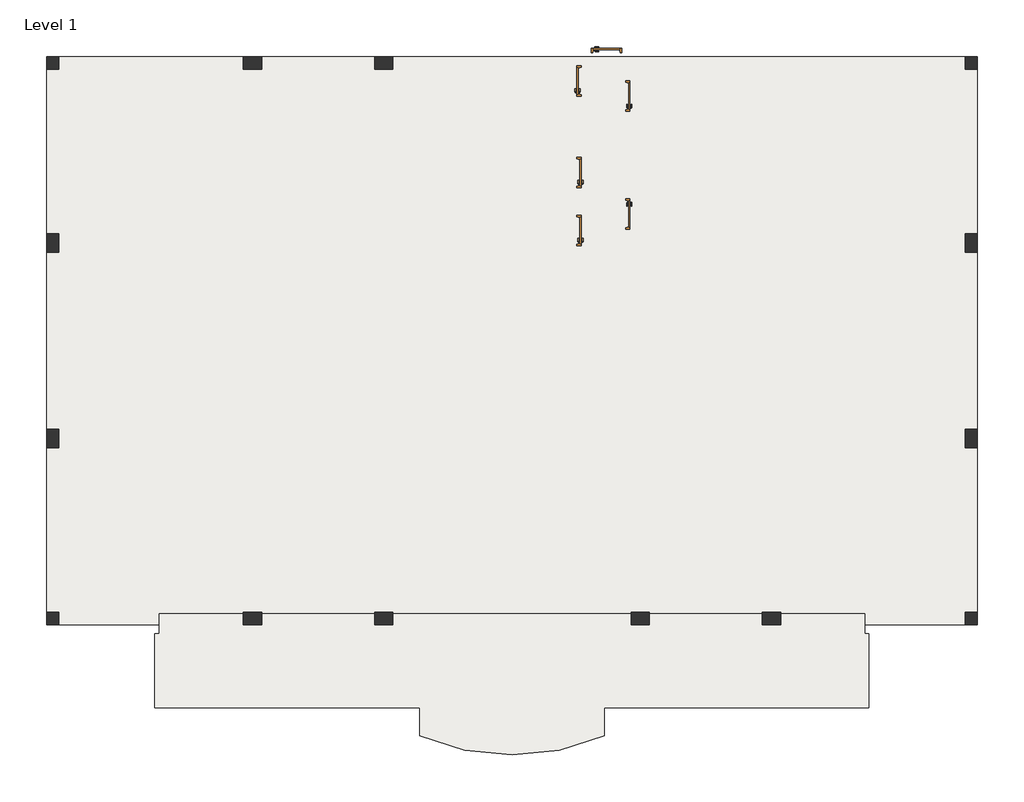
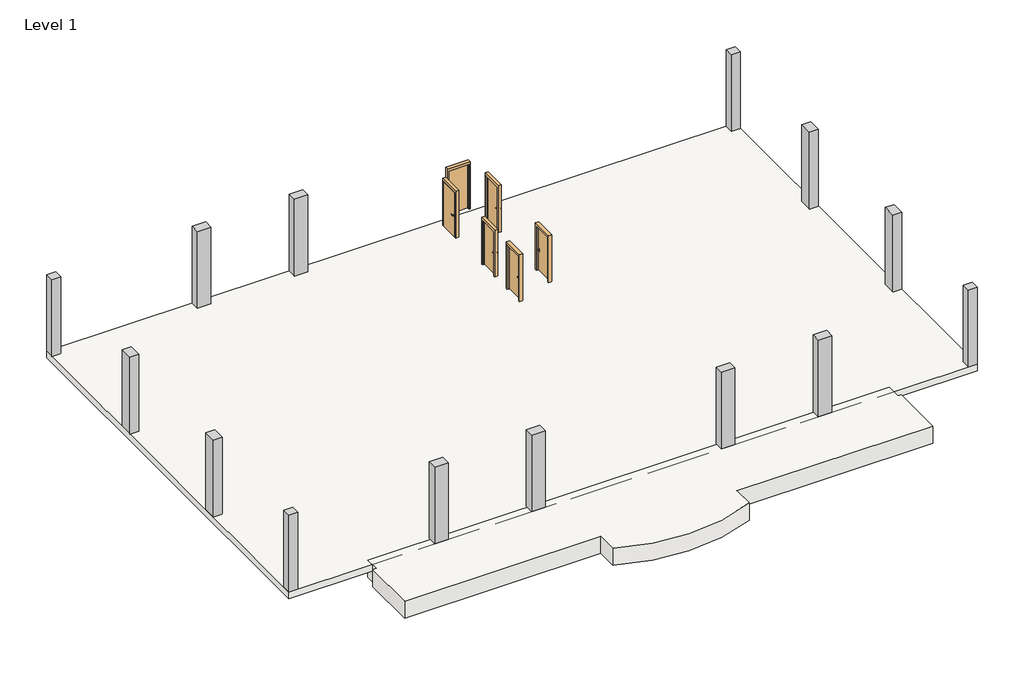
# One storey: 14 columns, 6 doors, 2 slabs.
"""IFC4 building model written with IfcOpenShell, lengths in millimetres."""

import ifcopenshell
import ifcopenshell.guid

model = None  # the IFC model being written
_history = None  # IfcOwnerHistory: only IFC2X3 demands one
_inside = {}  # id of a spatial element -> (the spatial element, [elements in it])
_under = {}  # id of a project, library or spatial element -> (it, [spatial elements below it])
_declared = {}  # id of a project -> (the project, [libraries it declares])
_typed = {}  # id of a type object -> (the type object, [elements of that type])
_made_of = {}  # id of a material, layer set ... -> (it, [elements and type objects made of it])


def new_model(schema):
    """Start an empty IFC model of exactly this schema.

    Asked for "IFC4X3", IfcOpenShell would pick the latest addendum, in which some entities
    have other attributes; the version numbers below select the first issue.
    IFC2X3 requires an IfcOwnerHistory on every rooted entity: one is made here for all.
    """
    global model, _history
    if schema == "IFC4X3":
        model = ifcopenshell.file(schema_version=(4, 3, 0, 0))
    else:
        model = ifcopenshell.file(schema=schema)
    _inside.clear()
    _under.clear()
    _declared.clear()
    _typed.clear()
    _made_of.clear()
    _history = None
    if model.schema == "IFC2X3":
        org = make("IfcOrganization", Name="unknown")
        user = make(
            "IfcPersonAndOrganization",
            ThePerson=make("IfcPerson", FamilyName="unknown"),
            TheOrganization=org,
        )
        app = make(
            "IfcApplication",
            ApplicationDeveloper=org,
            Version="unknown",
            ApplicationFullName="unknown",
            ApplicationIdentifier="unknown",
        )
        _history = make(
            "IfcOwnerHistory",
            OwningUser=user,
            OwningApplication=app,
            ChangeAction="ADDED",
            CreationDate=0,
        )
    return model


def make(cls, **values):
    """One entity of the class cls with the attributes given. An attribute that is None is left unset."""
    return model.create_entity(
        cls, **{name: value for name, value in values.items() if value is not None}
    )


def rooted(cls, **values):
    """An entity with a GlobalId (a new one), such as an element, a storey or a relation."""
    return make(cls, GlobalId=ifcopenshell.guid.new(), OwnerHistory=_history, **values)


def si_unit(unit_type, name, prefix=None):
    """IfcSIUnit, for example si_unit("LENGTHUNIT", "METRE", prefix="MILLI")."""
    return make("IfcSIUnit", UnitType=unit_type, Prefix=prefix, Name=name)


def assignment(units):
    """IfcUnitAssignment: the units of a project."""
    return None if units is None else make("IfcUnitAssignment", Units=units)


def point(xyz):
    """IfcCartesianPoint."""
    return None if xyz is None else make("IfcCartesianPoint", Coordinates=xyz)


def direction(xyz):
    """IfcDirection."""
    return None if xyz is None else make("IfcDirection", DirectionRatios=xyz)


def frame(location, z_axis=None, x_axis=None):
    """IfcAxis2Placement3D, a coordinate frame: its origin and axes. An axis left out is left unset."""
    return make(
        "IfcAxis2Placement3D",
        Location=point(location),
        Axis=direction(z_axis),
        RefDirection=direction(x_axis),
    )


def frame_2d(location, x_axis=None):
    """IfcAxis2Placement2D, a coordinate frame in the plane: its origin and x axis."""
    return make(
        "IfcAxis2Placement2D", Location=point(location), RefDirection=direction(x_axis)
    )


def origin():
    """The frame at (0, 0, 0) with its axes left unset."""
    return frame((0.0, 0.0, 0.0))


def origin_with_axes():
    """The frame at (0, 0, 0) with the z axis (0, 0, 1) and the x axis (1, 0, 0) written out."""
    return frame((0.0, 0.0, 0.0), z_axis=(0.0, 0.0, 1.0), x_axis=(1.0, 0.0, 0.0))


def place(relative_to, where):
    """IfcLocalPlacement: puts the frame where relative to a parent placement (None: the world)."""
    return make(
        "IfcLocalPlacement", PlacementRelTo=relative_to, RelativePlacement=where
    )


def context(
    kind, dimensions, precision=None, world=None, true_north=None, identifier=None
):
    """IfcGeometricRepresentationContext, for example the 3D "Model" context."""
    return make(
        "IfcGeometricRepresentationContext",
        ContextIdentifier=identifier,
        ContextType=kind,
        CoordinateSpaceDimension=dimensions,
        Precision=precision,
        WorldCoordinateSystem=world,
        TrueNorth=true_north,
    )


def project(units=None, contexts=None):
    """IfcProject with its units and contexts."""
    return rooted(
        "IfcProject",
        Name="project",
        RepresentationContexts=contexts,
        UnitsInContext=assignment(units),
    )


def spatial(cls, under=None, at=None, **own):
    """A site, building, storey or space (cls), placed at a placement, below another one or the project."""
    s = rooted(cls, ObjectPlacement=at, **own)
    if under is not None:
        _under.setdefault(under.id(), (under, []))[1].append(s)
    return s


def polyline(points):
    """IfcPolyline through the points."""
    return make("IfcPolyline", Points=[point(p) for p in points])


def circle_curve(where, radius):
    """IfcCircle in the frame where."""
    return make("IfcCircle", Position=where, Radius=radius)


def ellipse_curve(where, semi_axis1, semi_axis2):
    """IfcEllipse in the frame where."""
    return make(
        "IfcEllipse", Position=where, SemiAxis1=semi_axis1, SemiAxis2=semi_axis2
    )


def trimmed(basis, trim1, trim2, sense, master):
    """IfcTrimmedCurve: the piece of a basis curve between two trims."""
    return make(
        "IfcTrimmedCurve",
        BasisCurve=basis,
        Trim1=trim1,
        Trim2=trim2,
        SenseAgreement=sense,
        MasterRepresentation=master,
    )


def segment(curve, same_sense, transition):
    """IfcCompositeCurveSegment."""
    return make(
        "IfcCompositeCurveSegment",
        Transition=transition,
        SameSense=same_sense,
        ParentCurve=curve,
    )


def composite_curve(segments, self_intersect=None):
    """IfcCompositeCurve: segments joined end to end."""
    return make("IfcCompositeCurve", Segments=segments, SelfIntersect=self_intersect)


def outline(outer, holes=None, kind="AREA"):
    """IfcArbitraryClosedProfileDef: a profile drawn as a closed curve; with holes, ...WithVoids."""
    if holes is None:
        return make("IfcArbitraryClosedProfileDef", ProfileType=kind, OuterCurve=outer)
    return make(
        "IfcArbitraryProfileDefWithVoids",
        ProfileType=kind,
        OuterCurve=outer,
        InnerCurves=holes,
    )


def extrude(swept, where, along, depth):
    """IfcExtrudedAreaSolid: the profile swept, set in the frame where, extruded along a direction by depth."""
    return make(
        "IfcExtrudedAreaSolid",
        SweptArea=swept,
        Position=where,
        ExtrudedDirection=direction(along),
        Depth=depth,
    )


def faces_of(points, faces, orient=None, outer=None):
    """IfcFace entities. A face is a list of loops; a loop is a list of indices into points, from 0.

    orient and outer hold one flag for each loop. By default every Orientation is true, the
    first loop of a face is its IfcFaceOuterBound and the others are IfcFaceBound.
    """
    made = []
    for i, loops in enumerate(faces):
        bounds = []
        for j, loop in enumerate(loops):
            is_outer = j == 0 if outer is None else outer[i][j]
            bounds.append(
                make(
                    "IfcFaceOuterBound" if is_outer else "IfcFaceBound",
                    Bound=make("IfcPolyLoop", Polygon=[points[k] for k in loop]),
                    Orientation=True if orient is None else orient[i][j],
                )
            )
        made.append(make("IfcFace", Bounds=bounds))
    return made


def faceted_brep(points, faces, orient=None, outer=None, voids=None):
    """IfcFacetedBrep: a solid bounded by flat faces; with voids (closed shells), ...WithVoids."""
    shared = [point(p) for p in points]
    hull = make("IfcClosedShell", CfsFaces=faces_of(shared, faces, orient, outer))
    if voids is None:
        return make("IfcFacetedBrep", Outer=hull)
    return make(
        "IfcFacetedBrepWithVoids",
        Outer=hull,
        Voids=[
            make(cls, CfsFaces=faces_of(shared, fs, o, b)) for cls, fs, o, b in voids
        ],
    )


def shape(context_of_items, identifier, shape_type, items):
    """IfcShapeRepresentation: the items that make up one representation, for example the "Body"."""
    return make(
        "IfcShapeRepresentation",
        ContextOfItems=context_of_items,
        RepresentationIdentifier=identifier,
        RepresentationType=shape_type,
        Items=items,
    )


def source(mapping_origin, context_of_items, identifier, shape_type, items):
    """IfcRepresentationMap: a shape defined once, which mapped items show again and again."""
    return make(
        "IfcRepresentationMap",
        MappingOrigin=mapping_origin,
        MappedRepresentation=shape(context_of_items, identifier, shape_type, items),
    )


def transform(
    local_origin,
    x_axis=None,
    y_axis=None,
    z_axis=None,
    scale=None,
    scale2=None,
    scale3=None,
    uniform=True,
):
    """IfcCartesianTransformationOperator3D, or its non-uniform kind. x_axis, y_axis, z_axis: its Axis1, 2, 3."""
    if uniform:
        return make(
            "IfcCartesianTransformationOperator3D",
            Axis1=direction(x_axis),
            Axis2=direction(y_axis),
            LocalOrigin=point(local_origin),
            Scale=scale,
            Axis3=direction(z_axis),
        )
    return make(
        "IfcCartesianTransformationOperator3DnonUniform",
        Axis1=direction(x_axis),
        Axis2=direction(y_axis),
        LocalOrigin=point(local_origin),
        Scale=scale,
        Axis3=direction(z_axis),
        Scale2=scale2,
        Scale3=scale3,
    )


def mapped(mapping_source, mapping_target):
    """IfcMappedItem: shows the shape of a source again, moved by a transform."""
    return make(
        "IfcMappedItem", MappingSource=mapping_source, MappingTarget=mapping_target
    )


def made_of(thing, what):
    """Note that an element or type object is made of a material, layer set ...; save() writes the relation."""
    if what is not None:
        _made_of.setdefault(what.id(), (what, []))[1].append(thing)
    return thing


def element(
    cls,
    number,
    at=None,
    inside=None,
    cuts=None,
    type_object=None,
    material=None,
    context=None,
    identifier="Body",
    shape_type=None,
    held_by="IfcProductDefinitionShape",
    body=None,
    shapes=None,
    **own,
):
    """One element of the class cls, such as IfcWall. Its Tag is "e" and its number.

    at: its placement. inside: the storey or other place that contains it. cuts: it is an
    opening in that element (IfcRelVoidsElement). A single representation is given by context,
    identifier, shape_type and body (its items); several are given by shapes. held_by: the class
    of the entity that holds the representations. save() writes the other relations.
    """
    e = rooted(cls, Tag="e%d" % number, ObjectPlacement=at, **own)
    if body is not None:
        shapes = [shape(context, identifier, shape_type, body)]
    if shapes is not None:
        e.Representation = make(held_by, Representations=shapes)
    if inside is not None:
        _inside.setdefault(inside.id(), (inside, []))[1].append(e)
    if cuts is not None:
        rooted(
            "IfcRelVoidsElement", RelatingBuildingElement=cuts, RelatedOpeningElement=e
        )
    if type_object is not None:
        _typed.setdefault(type_object.id(), (type_object, []))[1].append(e)
    return made_of(e, material)


def aggregate(whole, parts):
    """IfcRelAggregates: a whole, such as a stair, and the parts it consists of."""
    return rooted("IfcRelAggregates", RelatingObject=whole, RelatedObjects=parts)


def save(model, path):
    """Write the relations noted so far, then the file.

    IfcRelAggregates (storeys below a building ...), IfcRelContainedInSpatialStructure (elements
    in a storey), IfcRelDefinesByType, IfcRelAssociatesMaterial and IfcRelDeclares: one each for
    every whole, place, type object, material and project.
    """
    for whole, parts in _under.values():
        aggregate(whole, parts)
    for where, things in _inside.values():
        rooted(
            "IfcRelContainedInSpatialStructure",
            RelatedElements=things,
            RelatingStructure=where,
        )
    for kind, things in _typed.values():
        rooted("IfcRelDefinesByType", RelatedObjects=things, RelatingType=kind)
    for what, things in _made_of.values():
        rooted("IfcRelAssociatesMaterial", RelatedObjects=things, RelatingMaterial=what)
    for by, libraries in _declared.values():
        rooted("IfcRelDeclares", RelatingContext=by, RelatedDefinitions=libraries)
    model.write(path)


def plane_surface(at):
    """IfcPlane: the flat surface through the origin of the frame at, square to its z axis."""
    return make("IfcPlane", Position=at)


def cylinder_surface(at, radius):
    """IfcCylindricalSurface: all points at the distance radius from the z axis of the frame at."""
    return make("IfcCylindricalSurface", Position=at, Radius=radius)


def revolved_surface(curve, axis_point, axis_direction):
    """IfcSurfaceOfRevolution: the curve turned about the line through axis_point along axis_direction."""
    return make(
        "IfcSurfaceOfRevolution",
        SweptCurve=make("IfcArbitraryOpenProfileDef", ProfileType="CURVE", Curve=curve),
        AxisPosition=make("IfcAxis1Placement", Location=point(axis_point), Axis=direction(axis_direction)),
    )


def advanced_brep(points, edges, surfaces, faces):
    """IfcAdvancedBrep: a solid bounded by faces that lie on surfaces and meet in shared edges.

    An edge is (start, end): straight between two places in points (the first is 0);
    or (start, end, curve); or (start, end, curve, False) where it runs against its curve.
    A face is (place in surfaces, loops), or (place, loops, False) where it looks against
    its surface's normal. A loop lists edges by number (the first is 1), with a minus sign
    where the edge is run from its end to its start. The first loop is the outer one.
    """
    corners = [point(p) for p in points]
    vertices = [make("IfcVertexPoint", VertexGeometry=c) for c in corners]
    made = []
    for start, end, *more in edges:
        made.append(
            make(
                "IfcEdgeCurve",
                EdgeStart=vertices[start],
                EdgeEnd=vertices[end],
                EdgeGeometry=more[0] if more else make("IfcPolyline", Points=[corners[start], corners[end]]),
                SameSense=more[1] if len(more) > 1 else True,
            )
        )
    hull = []
    for where, loops, *sense in faces:
        bounds = []
        for j, loop in enumerate(loops):
            ring = [make("IfcOrientedEdge", EdgeElement=made[abs(k) - 1], Orientation=k > 0) for k in loop]
            bounds.append(
                make(
                    "IfcFaceOuterBound" if j == 0 else "IfcFaceBound",
                    Bound=make("IfcEdgeLoop", EdgeList=ring),
                    Orientation=True,
                )
            )
        hull.append(make("IfcAdvancedFace", Bounds=bounds, FaceSurface=surfaces[where], SameSense=sense[0] if sense else True))
    return make("IfcAdvancedBrep", Outer=make("IfcClosedShell", CfsFaces=hull))


def door_e56c0533(model_context):
    return source(origin(), model_context, "Body", "SolidModel", [
        advanced_brep(
        [(-392.190625, 76.1375, 1016.0), (-372.190625, 76.1375, 1016.0), (-372.190625, 46.1375, 1016.0), (-392.190625, 46.1375, 1016.0), (-367.190625, 41.1375, 1016.0), (-367.190625, 21.1375, 1016.0), (-262.190625, 21.1375, 1016.0), (-262.190625, 41.1375, 1016.0)],
        [
            (0, 1, circle_curve(frame((-382.190625, 76.1375, 1016.0), z_axis=(0.0, 1.0, 0.0), x_axis=(1.0, 0.0, 0.0)), 10.0)),
            (1, 0, circle_curve(frame((-382.190625, 76.1375, 1016.0), z_axis=(0.0, 1.0, 0.0), x_axis=(1.0, 0.0, 0.0)), 10.0)),
            (1, 2),
            (2, 3, circle_curve(frame((-382.190625, 46.1375, 1016.0), z_axis=(0.0, 1.0, 0.0), x_axis=(1.0, 0.0, 0.0)), 10.0)),
            (3, 0),
            (3, 2, circle_curve(frame((-382.190625, 46.1375, 1016.0), z_axis=(0.0, 1.0, 0.0), x_axis=(1.0, 0.0, 0.0)), 10.0)),
            (4, 5, circle_curve(frame((-367.190625, 31.1375, 1016.0), z_axis=(-1.0, 0.0, 0.0), x_axis=(0.0, 1.0, 0.0)), 10.0)),
            (5, 3, circle_curve(frame((-367.190625, 46.1375, 1016.0), z_axis=(0.0, 0.0, -1.0), x_axis=(-1.0, 0.0, 0.0)), 25.0)),
            (2, 4, circle_curve(frame((-367.190625, 46.1375, 1016.0), z_axis=(0.0, 0.0, 1.0), x_axis=(-1.0, 0.0, 0.0)), 5.0)),
            (5, 4, circle_curve(frame((-367.190625, 31.1375, 1016.0), z_axis=(-1.0, 0.0, 0.0), x_axis=(0.0, 1.0, 0.0)), 10.0)),
            (6, 7, circle_curve(frame((-262.190625, 31.1375, 1016.0), z_axis=(1.0, 0.0, 0.0), x_axis=(0.0, 1.0, 0.0)), 10.0)),
            (7, 6, circle_curve(frame((-262.190625, 31.1375, 1016.0), z_axis=(1.0, 0.0, 0.0), x_axis=(0.0, 1.0, 0.0)), 10.0)),
            (4, 7),
            (6, 5),
        ],
        [
            plane_surface(frame((-382.190625, 76.1375, 1016.0), z_axis=(0.0, 1.0, 0.0), x_axis=(0.0, 0.0, 1.0))),
            cylinder_surface(frame((-382.190625, 76.1375, 1016.0), z_axis=(0.0, 1.0, 0.0), x_axis=(1.0, 0.0, 0.0)), 10.0),
            revolved_surface(trimmed(ellipse_curve(frame((-382.190625, 46.1375, 1016.0), z_axis=(0.0, -1.0, 0.0), x_axis=(1.0, 0.0, 0.0)), 10.0, 10.0), [point((-392.190625, 46.1375, 1016.0))], [point((-372.190625, 46.1375, 1016.0))], True, "CARTESIAN"), (-367.190625, 46.1375, 1016.0), (0.0, 0.0, -1.0)),
            revolved_surface(trimmed(ellipse_curve(frame((-382.190625, 46.1375, 1016.0), z_axis=(0.0, -1.0, 0.0), x_axis=(1.0, 0.0, 0.0)), 10.0, 10.0), [point((-372.190625, 46.1375, 1016.0))], [point((-392.190625, 46.1375, 1016.0))], True, "CARTESIAN"), (-367.190625, 46.1375, 1016.0), (0.0, 0.0, -1.0)),
            plane_surface(frame((-262.190625, 31.1375, 1016.0), z_axis=(1.0, 0.0, 0.0), x_axis=(0.0, 0.0, 1.0))),
            cylinder_surface(frame((-367.190625, 31.1375, 1016.0), z_axis=(-1.0, 0.0, 0.0), x_axis=(0.0, 1.0, 0.0)), 10.0),
        ],
        [
            (0, [[1, 2]]),
            (1, [[3, 4, 5, -2]]),
            (1, [[-5, 6, -3, -1]]),
            (2, [[7, 8, -4, 9]]),
            (3, [[10, -9, -6, -8]]),
            (4, [[11, 12]]),
            (5, [[13, -11, 14, -7]]),
            (5, [[-14, -12, -13, -10]]),
        ],
    ),
        extrude(outline(composite_curve([segment(trimmed(circle_curve(frame_2d((1016.0, -384.690625)), 30.0), [point((1016.0, -414.690625))], [point((1016.0, -354.690625))], False, "CARTESIAN"), True, "CONTINUOUS"), segment(trimmed(circle_curve(frame_2d((1016.0, -384.690625)), 30.0), [point((1016.0, -354.690625))], [point((1016.0, -414.690625))], False, "CARTESIAN"), True, "CONTINUOUS")], self_intersect=False)), frame((0.0, 76.1375, 0.0), z_axis=(0.0, 1.0, 0.0), x_axis=(0.0, 0.0, 1.0)), (0.0, 0.0, 1.0), 8.0),
        advanced_brep(
        [(-392.190625, 136.5875, 1016.0), (-372.190625, 136.5875, 1016.0), (-392.190625, 166.5875, 1016.0), (-372.190625, 166.5875, 1016.0), (-367.190625, 171.5875, 1016.0), (-367.190625, 191.5875, 1016.0), (-262.190625, 191.5875, 1016.0), (-262.190625, 171.5875, 1016.0)],
        [
            (0, 1, circle_curve(frame((-382.190625, 136.5875, 1016.0), z_axis=(0.0, -1.0, 0.0), x_axis=(1.0, 0.0, 0.0)), 10.0)),
            (1, 0, circle_curve(frame((-382.190625, 136.5875, 1016.0), z_axis=(0.0, -1.0, 0.0), x_axis=(1.0, 0.0, 0.0)), 10.0)),
            (0, 2),
            (2, 3, circle_curve(frame((-382.190625, 166.5875, 1016.0), z_axis=(0.0, -1.0, 0.0), x_axis=(1.0, 0.0, 0.0)), 10.0)),
            (3, 1),
            (3, 2, circle_curve(frame((-382.190625, 166.5875, 1016.0), z_axis=(0.0, -1.0, 0.0), x_axis=(1.0, 0.0, 0.0)), 10.0)),
            (4, 3, circle_curve(frame((-367.190625, 166.5875, 1016.0), z_axis=(0.0, 0.0, 1.0), x_axis=(-1.0, 0.0, 0.0)), 5.0)),
            (2, 5, circle_curve(frame((-367.190625, 166.5875, 1016.0), z_axis=(0.0, 0.0, -1.0), x_axis=(-1.0, 0.0, 0.0)), 25.0)),
            (5, 4, circle_curve(frame((-367.190625, 181.5875, 1016.0), z_axis=(-1.0, 0.0, 0.0), x_axis=(0.0, -1.0, 0.0)), 10.0)),
            (4, 5, circle_curve(frame((-367.190625, 181.5875, 1016.0), z_axis=(-1.0, 0.0, 0.0), x_axis=(0.0, -1.0, 0.0)), 10.0)),
            (6, 7, circle_curve(frame((-262.190625, 181.5875, 1016.0), z_axis=(1.0, 0.0, 0.0), x_axis=(0.0, -1.0, 0.0)), 10.0)),
            (7, 6, circle_curve(frame((-262.190625, 181.5875, 1016.0), z_axis=(1.0, 0.0, 0.0), x_axis=(0.0, -1.0, 0.0)), 10.0)),
            (5, 6),
            (7, 4),
        ],
        [
            plane_surface(frame((-382.190625, 136.5875, 1016.0), z_axis=(0.0, -1.0, 0.0), x_axis=(0.0, 0.0, 1.0))),
            cylinder_surface(frame((-382.190625, 136.5875, 1016.0), z_axis=(0.0, -1.0, 0.0), x_axis=(1.0, 0.0, 0.0)), 10.0),
            revolved_surface(trimmed(ellipse_curve(frame((-382.190625, 166.5875, 1016.0), z_axis=(0.0, -1.0, 0.0), x_axis=(1.0, 0.0, 0.0)), 10.0, 10.0), [point((-392.190625, 166.5875, 1016.0))], [point((-372.190625, 166.5875, 1016.0))], True, "CARTESIAN"), (-367.190625, 166.5875, 1016.0), (0.0, 0.0, -1.0)),
            revolved_surface(trimmed(ellipse_curve(frame((-382.190625, 166.5875, 1016.0), z_axis=(0.0, -1.0, 0.0), x_axis=(1.0, 0.0, 0.0)), 10.0, 10.0), [point((-372.190625, 166.5875, 1016.0))], [point((-392.190625, 166.5875, 1016.0))], True, "CARTESIAN"), (-367.190625, 166.5875, 1016.0), (0.0, 0.0, -1.0)),
            plane_surface(frame((-262.190625, 181.5875, 1016.0), z_axis=(1.0, 0.0, 0.0), x_axis=(0.0, 0.0, 1.0))),
            cylinder_surface(frame((-367.190625, 181.5875, 1016.0), z_axis=(-1.0, 0.0, 0.0), x_axis=(0.0, -1.0, 0.0)), 10.0),
        ],
        [
            (0, [[1, 2]]),
            (1, [[-1, 3, 4, 5]]),
            (1, [[-2, -5, 6, -3]]),
            (2, [[7, -4, 8, 9]]),
            (3, [[-8, -6, -7, 10]]),
            (4, [[11, 12]]),
            (5, [[-9, 13, -12, 14]]),
            (5, [[-10, -14, -11, -13]]),
        ],
    ),
        extrude(outline(composite_curve([segment(trimmed(circle_curve(frame_2d((1016.0, -384.690625)), 30.0), [point((1016.0, -414.690625))], [point((1016.0, -354.690625))], False, "CARTESIAN"), True, "CONTINUOUS"), segment(trimmed(circle_curve(frame_2d((1016.0, -384.690625)), 30.0), [point((1016.0, -354.690625))], [point((1016.0, -414.690625))], False, "CARTESIAN"), True, "CONTINUOUS")], self_intersect=False)), frame((0.0, 128.5875, 0.0), z_axis=(0.0, 1.0, 0.0), x_axis=(0.0, 0.0, 1.0)), (0.0, 0.0, 1.0), 8.0),
        faceted_brep([(457.2, 79.375, 0.0), (457.2, 128.5875, 0.0), (508.0, 128.5875, 0.0), (508.0, -17.4625, 0.0), (457.2, -17.4625, 0.0), (457.2, 31.75, 0.0), (441.325, 31.75, 0.0), (441.325, 79.375, 0.0), (457.2, 79.375, 2133.6), (457.2, 128.5875, 2133.6), (-457.2, 128.5875, 2133.6), (-457.2, 128.5875, 0.0), (-508.0, 128.5875, 0.0), (-508.0, 128.5875, 2235.2), (508.0, 128.5875, 2235.2), (508.0, -17.4625, 2235.2), (-508.0, -17.4625, 2235.2), (-508.0, -17.4625, 0.0), (-457.2, -17.4625, 0.0), (-457.2, -17.4625, 2133.6), (457.2, -17.4625, 2133.6), (457.2, 31.75, 2133.6), (-457.2, 31.75, 2133.6), (-457.2, 31.75, 0.0), (-441.325, 31.75, 0.0), (-441.325, 31.75, 2117.725), (441.325, 31.75, 2117.725), (441.325, 79.375, 2117.725), (-441.325, 79.375, 2117.725), (-441.325, 79.375, 0.0), (-457.2, 79.375, 0.0), (-457.2, 79.375, 2133.6)], [[[0, 1, 2, 3, 4, 5, 6, 7]], [[1, 0, 8, 9]], [[2, 1, 9, 10, 11, 12, 13, 14]], [[3, 2, 14, 15]], [[4, 3, 15, 16, 17, 18, 19, 20]], [[5, 4, 20, 21]], [[6, 5, 21, 22, 23, 24, 25, 26]], [[7, 6, 26, 27]], [[0, 7, 27, 28, 29, 30, 31, 8]], [[9, 8, 31, 10]], [[20, 19, 22, 21]], [[26, 25, 28, 27]], [[12, 11, 30, 29, 24, 23, 18, 17]], [[11, 10, 31, 30]], [[13, 12, 17, 16]], [[19, 18, 23, 22]], [[25, 24, 29, 28]], [[15, 14, 13, 16]]]),
        extrude(outline(polyline([(457.2, 84.1375), (-457.2, 84.1375), (-457.2, 128.5875), (457.2, 128.5875), (457.2, 84.1375)])), origin_with_axes(), (0.0, 0.0, 1.0), 2133.6),
    ])


def door_9f6fe377(model_context):
    return source(origin(), model_context, "Body", "SolidModel", [
        advanced_brep(
        [(-392.190625, -25.3375, 1016.0), (-372.190625, -25.3375, 1016.0), (-392.190625, 4.6625, 1016.0), (-372.190625, 4.6625, 1016.0), (-367.190625, 9.6625, 1016.0), (-367.190625, 29.6625, 1016.0), (-262.190625, 29.6625, 1016.0), (-262.190625, 9.6625, 1016.0)],
        [
            (0, 1, circle_curve(frame((-382.190625, -25.3375, 1016.0), z_axis=(0.0, -1.0, 0.0), x_axis=(1.0, 0.0, 0.0)), 10.0)),
            (1, 0, circle_curve(frame((-382.190625, -25.3375, 1016.0), z_axis=(0.0, -1.0, 0.0), x_axis=(1.0, 0.0, 0.0)), 10.0)),
            (0, 2),
            (2, 3, circle_curve(frame((-382.190625, 4.6625, 1016.0), z_axis=(0.0, -1.0, 0.0), x_axis=(1.0, 0.0, 0.0)), 10.0)),
            (3, 1),
            (3, 2, circle_curve(frame((-382.190625, 4.6625, 1016.0), z_axis=(0.0, -1.0, 0.0), x_axis=(1.0, 0.0, 0.0)), 10.0)),
            (4, 3, circle_curve(frame((-367.190625, 4.6625, 1016.0), z_axis=(0.0, 0.0, 1.0), x_axis=(-1.0, 0.0, 0.0)), 5.0)),
            (2, 5, circle_curve(frame((-367.190625, 4.6625, 1016.0), z_axis=(0.0, 0.0, -1.0), x_axis=(-1.0, 0.0, 0.0)), 25.0)),
            (5, 4, circle_curve(frame((-367.190625, 19.6625, 1016.0), z_axis=(-1.0, 0.0, 0.0), x_axis=(0.0, -1.0, 0.0)), 10.0)),
            (4, 5, circle_curve(frame((-367.190625, 19.6625, 1016.0), z_axis=(-1.0, 0.0, 0.0), x_axis=(0.0, -1.0, 0.0)), 10.0)),
            (6, 7, circle_curve(frame((-262.190625, 19.6625, 1016.0), z_axis=(1.0, 0.0, 0.0), x_axis=(0.0, -1.0, 0.0)), 10.0)),
            (7, 6, circle_curve(frame((-262.190625, 19.6625, 1016.0), z_axis=(1.0, 0.0, 0.0), x_axis=(0.0, -1.0, 0.0)), 10.0)),
            (5, 6),
            (7, 4),
        ],
        [
            plane_surface(frame((-382.190625, -25.3375, 1016.0), z_axis=(0.0, -1.0, 0.0), x_axis=(0.0, 0.0, 1.0))),
            cylinder_surface(frame((-382.190625, -25.3375, 1016.0), z_axis=(0.0, -1.0, 0.0), x_axis=(1.0, 0.0, 0.0)), 10.0),
            revolved_surface(trimmed(ellipse_curve(frame((-382.190625, 4.6625, 1016.0), z_axis=(0.0, -1.0, 0.0), x_axis=(1.0, 0.0, 0.0)), 10.0, 10.0), [point((-392.190625, 4.6625, 1016.0))], [point((-372.190625, 4.6625, 1016.0))], True, "CARTESIAN"), (-367.190625, 4.6625, 1016.0), (0.0, 0.0, -1.0)),
            revolved_surface(trimmed(ellipse_curve(frame((-382.190625, 4.6625, 1016.0), z_axis=(0.0, -1.0, 0.0), x_axis=(1.0, 0.0, 0.0)), 10.0, 10.0), [point((-372.190625, 4.6625, 1016.0))], [point((-392.190625, 4.6625, 1016.0))], True, "CARTESIAN"), (-367.190625, 4.6625, 1016.0), (0.0, 0.0, -1.0)),
            plane_surface(frame((-262.190625, 19.6625, 1016.0), z_axis=(1.0, 0.0, 0.0), x_axis=(0.0, 0.0, 1.0))),
            cylinder_surface(frame((-367.190625, 19.6625, 1016.0), z_axis=(-1.0, 0.0, 0.0), x_axis=(0.0, -1.0, 0.0)), 10.0),
        ],
        [
            (0, [[1, 2]]),
            (1, [[-1, 3, 4, 5]]),
            (1, [[-2, -5, 6, -3]]),
            (2, [[7, -4, 8, 9]]),
            (3, [[-8, -6, -7, 10]]),
            (4, [[11, 12]]),
            (5, [[-9, 13, -12, 14]]),
            (5, [[-10, -14, -11, -13]]),
        ],
    ),
        extrude(outline(composite_curve([segment(trimmed(circle_curve(frame_2d((1016.0, -384.690625)), 30.0), [point((1016.0, -414.690625))], [point((1016.0, -354.690625))], False, "CARTESIAN"), True, "CONTINUOUS"), segment(trimmed(circle_curve(frame_2d((1016.0, -384.690625)), 30.0), [point((1016.0, -354.690625))], [point((1016.0, -414.690625))], False, "CARTESIAN"), True, "CONTINUOUS")], self_intersect=False)), frame((0.0, -33.3375, 0.0), z_axis=(0.0, 1.0, 0.0), x_axis=(0.0, 0.0, 1.0)), (0.0, 0.0, 1.0), 8.0),
        advanced_brep(
        [(-392.190625, -85.7875, 1016.0), (-372.190625, -85.7875, 1016.0), (-372.190625, -115.7875, 1016.0), (-392.190625, -115.7875, 1016.0), (-367.190625, -120.7875, 1016.0), (-367.190625, -140.7875, 1016.0), (-262.190625, -140.7875, 1016.0), (-262.190625, -120.7875, 1016.0)],
        [
            (0, 1, circle_curve(frame((-382.190625, -85.7875, 1016.0), z_axis=(0.0, 1.0, 0.0), x_axis=(1.0, 0.0, 0.0)), 10.0)),
            (1, 0, circle_curve(frame((-382.190625, -85.7875, 1016.0), z_axis=(0.0, 1.0, 0.0), x_axis=(1.0, 0.0, 0.0)), 10.0)),
            (1, 2),
            (2, 3, circle_curve(frame((-382.190625, -115.7875, 1016.0), z_axis=(0.0, 1.0, 0.0), x_axis=(1.0, 0.0, 0.0)), 10.0)),
            (3, 0),
            (3, 2, circle_curve(frame((-382.190625, -115.7875, 1016.0), z_axis=(0.0, 1.0, 0.0), x_axis=(1.0, 0.0, 0.0)), 10.0)),
            (4, 5, circle_curve(frame((-367.190625, -130.7875, 1016.0), z_axis=(-1.0, 0.0, 0.0), x_axis=(0.0, 1.0, 0.0)), 10.0)),
            (5, 3, circle_curve(frame((-367.190625, -115.7875, 1016.0), z_axis=(0.0, 0.0, -1.0), x_axis=(-1.0, 0.0, 0.0)), 25.0)),
            (2, 4, circle_curve(frame((-367.190625, -115.7875, 1016.0), z_axis=(0.0, 0.0, 1.0), x_axis=(-1.0, 0.0, 0.0)), 5.0)),
            (5, 4, circle_curve(frame((-367.190625, -130.7875, 1016.0), z_axis=(-1.0, 0.0, 0.0), x_axis=(0.0, 1.0, 0.0)), 10.0)),
            (6, 7, circle_curve(frame((-262.190625, -130.7875, 1016.0), z_axis=(1.0, 0.0, 0.0), x_axis=(0.0, 1.0, 0.0)), 10.0)),
            (7, 6, circle_curve(frame((-262.190625, -130.7875, 1016.0), z_axis=(1.0, 0.0, 0.0), x_axis=(0.0, 1.0, 0.0)), 10.0)),
            (4, 7),
            (6, 5),
        ],
        [
            plane_surface(frame((-382.190625, -85.7875, 1016.0), z_axis=(0.0, 1.0, 0.0), x_axis=(0.0, 0.0, 1.0))),
            cylinder_surface(frame((-382.190625, -85.7875, 1016.0), z_axis=(0.0, 1.0, 0.0), x_axis=(1.0, 0.0, 0.0)), 10.0),
            revolved_surface(trimmed(ellipse_curve(frame((-382.190625, -115.7875, 1016.0), z_axis=(0.0, -1.0, 0.0), x_axis=(1.0, 0.0, 0.0)), 10.0, 10.0), [point((-392.190625, -115.7875, 1016.0))], [point((-372.190625, -115.7875, 1016.0))], True, "CARTESIAN"), (-367.190625, -115.7875, 1016.0), (0.0, 0.0, -1.0)),
            revolved_surface(trimmed(ellipse_curve(frame((-382.190625, -115.7875, 1016.0), z_axis=(0.0, -1.0, 0.0), x_axis=(1.0, 0.0, 0.0)), 10.0, 10.0), [point((-372.190625, -115.7875, 1016.0))], [point((-392.190625, -115.7875, 1016.0))], True, "CARTESIAN"), (-367.190625, -115.7875, 1016.0), (0.0, 0.0, -1.0)),
            plane_surface(frame((-262.190625, -130.7875, 1016.0), z_axis=(1.0, 0.0, 0.0), x_axis=(0.0, 0.0, 1.0))),
            cylinder_surface(frame((-367.190625, -130.7875, 1016.0), z_axis=(-1.0, 0.0, 0.0), x_axis=(0.0, 1.0, 0.0)), 10.0),
        ],
        [
            (0, [[1, 2]]),
            (1, [[3, 4, 5, -2]]),
            (1, [[-5, 6, -3, -1]]),
            (2, [[7, 8, -4, 9]]),
            (3, [[10, -9, -6, -8]]),
            (4, [[11, 12]]),
            (5, [[13, -11, 14, -7]]),
            (5, [[-14, -12, -13, -10]]),
        ],
    ),
        extrude(outline(composite_curve([segment(trimmed(circle_curve(frame_2d((1016.0, -384.690625)), 30.0), [point((1016.0, -414.690625))], [point((1016.0, -354.690625))], False, "CARTESIAN"), True, "CONTINUOUS"), segment(trimmed(circle_curve(frame_2d((1016.0, -384.690625)), 30.0), [point((1016.0, -354.690625))], [point((1016.0, -414.690625))], False, "CARTESIAN"), True, "CONTINUOUS")], self_intersect=False)), frame((0.0, -85.7875, 0.0), z_axis=(0.0, 1.0, 0.0), x_axis=(0.0, 0.0, 1.0)), (0.0, 0.0, 1.0), 8.0),
        faceted_brep([(457.2, -28.575, 0.0), (441.325, -28.575, 0.0), (441.325, 19.05, 0.0), (457.2, 19.05, 0.0), (457.2, 68.2625, 0.0), (508.0, 68.2625, 0.0), (508.0, -77.7875, 0.0), (457.2, -77.7875, 0.0), (457.2, -77.7875, 2133.6), (457.2, -28.575, 2133.6), (508.0, -77.7875, 2235.2), (-508.0, -77.7875, 2235.2), (-508.0, -77.7875, 0.0), (-457.2, -77.7875, 0.0), (-457.2, -77.7875, 2133.6), (508.0, 68.2625, 2235.2), (457.2, 68.2625, 2133.6), (-457.2, 68.2625, 2133.6), (-457.2, 68.2625, 0.0), (-508.0, 68.2625, 0.0), (-508.0, 68.2625, 2235.2), (457.2, 19.05, 2133.6), (441.325, 19.05, 2117.725), (-441.325, 19.05, 2117.725), (-441.325, 19.05, 0.0), (-457.2, 19.05, 0.0), (-457.2, 19.05, 2133.6), (441.325, -28.575, 2117.725), (-457.2, -28.575, 2133.6), (-457.2, -28.575, 0.0), (-441.325, -28.575, 0.0), (-441.325, -28.575, 2117.725)], [[[0, 1, 2, 3, 4, 5, 6, 7]], [[7, 8, 9, 0]], [[6, 10, 11, 12, 13, 14, 8, 7]], [[5, 15, 10, 6]], [[4, 16, 17, 18, 19, 20, 15, 5]], [[3, 21, 16, 4]], [[2, 22, 23, 24, 25, 26, 21, 3]], [[1, 27, 22, 2]], [[0, 9, 28, 29, 30, 31, 27, 1]], [[8, 14, 28, 9]], [[16, 21, 26, 17]], [[22, 27, 31, 23]], [[12, 19, 18, 25, 24, 30, 29, 13]], [[13, 29, 28, 14]], [[11, 20, 19, 12]], [[17, 26, 25, 18]], [[23, 31, 30, 24]], [[15, 20, 11, 10]]]),
        extrude(outline(polyline([(457.2, -33.3375), (457.2, -77.7875), (-457.2, -77.7875), (-457.2, -33.3375), (457.2, -33.3375)])), origin_with_axes(), (0.0, 0.0, 1.0), 2133.6),
    ])


def door_87fe937e(model_context):
    return source(origin(), model_context, "Body", "SolidModel", [
        advanced_brep(
        [(-392.190625, 25.3375, 1016.0), (-372.190625, 25.3375, 1016.0), (-372.190625, -4.6625, 1016.0), (-392.190625, -4.6625, 1016.0), (-367.190625, -9.6625, 1016.0), (-367.190625, -29.6625, 1016.0), (-262.190625, -29.6625, 1016.0), (-262.190625, -9.6625, 1016.0)],
        [
            (0, 1, circle_curve(frame((-382.190625, 25.3375, 1016.0), z_axis=(0.0, 1.0, 0.0), x_axis=(1.0, 0.0, 0.0)), 10.0)),
            (1, 0, circle_curve(frame((-382.190625, 25.3375, 1016.0), z_axis=(0.0, 1.0, 0.0), x_axis=(1.0, 0.0, 0.0)), 10.0)),
            (1, 2),
            (2, 3, circle_curve(frame((-382.190625, -4.6625, 1016.0), z_axis=(0.0, 1.0, 0.0), x_axis=(1.0, 0.0, 0.0)), 10.0)),
            (3, 0),
            (3, 2, circle_curve(frame((-382.190625, -4.6625, 1016.0), z_axis=(0.0, 1.0, 0.0), x_axis=(1.0, 0.0, 0.0)), 10.0)),
            (4, 5, circle_curve(frame((-367.190625, -19.6625, 1016.0), z_axis=(-1.0, 0.0, 0.0), x_axis=(0.0, 1.0, 0.0)), 10.0)),
            (5, 3, circle_curve(frame((-367.190625, -4.6625, 1016.0), z_axis=(0.0, 0.0, -1.0), x_axis=(-1.0, 0.0, 0.0)), 25.0)),
            (2, 4, circle_curve(frame((-367.190625, -4.6625, 1016.0), z_axis=(0.0, 0.0, 1.0), x_axis=(-1.0, 0.0, 0.0)), 5.0)),
            (5, 4, circle_curve(frame((-367.190625, -19.6625, 1016.0), z_axis=(-1.0, 0.0, 0.0), x_axis=(0.0, 1.0, 0.0)), 10.0)),
            (6, 7, circle_curve(frame((-262.190625, -19.6625, 1016.0), z_axis=(1.0, 0.0, 0.0), x_axis=(0.0, 1.0, 0.0)), 10.0)),
            (7, 6, circle_curve(frame((-262.190625, -19.6625, 1016.0), z_axis=(1.0, 0.0, 0.0), x_axis=(0.0, 1.0, 0.0)), 10.0)),
            (4, 7),
            (6, 5),
        ],
        [
            plane_surface(frame((-382.190625, 25.3375, 1016.0), z_axis=(0.0, 1.0, 0.0), x_axis=(0.0, 0.0, 1.0))),
            cylinder_surface(frame((-382.190625, 25.3375, 1016.0), z_axis=(0.0, 1.0, 0.0), x_axis=(1.0, 0.0, 0.0)), 10.0),
            revolved_surface(trimmed(ellipse_curve(frame((-382.190625, -4.6625, 1016.0), z_axis=(0.0, -1.0, 0.0), x_axis=(1.0, 0.0, 0.0)), 10.0, 10.0), [point((-392.190625, -4.6625, 1016.0))], [point((-372.190625, -4.6625, 1016.0))], True, "CARTESIAN"), (-367.190625, -4.6625, 1016.0), (0.0, 0.0, -1.0)),
            revolved_surface(trimmed(ellipse_curve(frame((-382.190625, -4.6625, 1016.0), z_axis=(0.0, -1.0, 0.0), x_axis=(1.0, 0.0, 0.0)), 10.0, 10.0), [point((-372.190625, -4.6625, 1016.0))], [point((-392.190625, -4.6625, 1016.0))], True, "CARTESIAN"), (-367.190625, -4.6625, 1016.0), (0.0, 0.0, -1.0)),
            plane_surface(frame((-262.190625, -19.6625, 1016.0), z_axis=(1.0, 0.0, 0.0), x_axis=(0.0, 0.0, 1.0))),
            cylinder_surface(frame((-367.190625, -19.6625, 1016.0), z_axis=(-1.0, 0.0, 0.0), x_axis=(0.0, 1.0, 0.0)), 10.0),
        ],
        [
            (0, [[1, 2]]),
            (1, [[3, 4, 5, -2]]),
            (1, [[-5, 6, -3, -1]]),
            (2, [[7, 8, -4, 9]]),
            (3, [[10, -9, -6, -8]]),
            (4, [[11, 12]]),
            (5, [[13, -11, 14, -7]]),
            (5, [[-14, -12, -13, -10]]),
        ],
    ),
        extrude(outline(composite_curve([segment(trimmed(circle_curve(frame_2d((1016.0, -384.690625)), 30.0), [point((1016.0, -414.690625))], [point((1016.0, -354.690625))], False, "CARTESIAN"), True, "CONTINUOUS"), segment(trimmed(circle_curve(frame_2d((1016.0, -384.690625)), 30.0), [point((1016.0, -354.690625))], [point((1016.0, -414.690625))], False, "CARTESIAN"), True, "CONTINUOUS")], self_intersect=False)), frame((0.0, 25.3375, 0.0), z_axis=(0.0, 1.0, 0.0), x_axis=(0.0, 0.0, 1.0)), (0.0, 0.0, 1.0), 8.0),
        advanced_brep(
        [(-392.190625, 85.7875, 1016.0), (-372.190625, 85.7875, 1016.0), (-392.190625, 115.7875, 1016.0), (-372.190625, 115.7875, 1016.0), (-367.190625, 120.7875, 1016.0), (-367.190625, 140.7875, 1016.0), (-262.190625, 140.7875, 1016.0), (-262.190625, 120.7875, 1016.0)],
        [
            (0, 1, circle_curve(frame((-382.190625, 85.7875, 1016.0), z_axis=(0.0, -1.0, 0.0), x_axis=(1.0, 0.0, 0.0)), 10.0)),
            (1, 0, circle_curve(frame((-382.190625, 85.7875, 1016.0), z_axis=(0.0, -1.0, 0.0), x_axis=(1.0, 0.0, 0.0)), 10.0)),
            (0, 2),
            (2, 3, circle_curve(frame((-382.190625, 115.7875, 1016.0), z_axis=(0.0, -1.0, 0.0), x_axis=(1.0, 0.0, 0.0)), 10.0)),
            (3, 1),
            (3, 2, circle_curve(frame((-382.190625, 115.7875, 1016.0), z_axis=(0.0, -1.0, 0.0), x_axis=(1.0, 0.0, 0.0)), 10.0)),
            (4, 3, circle_curve(frame((-367.190625, 115.7875, 1016.0), z_axis=(0.0, 0.0, 1.0), x_axis=(-1.0, 0.0, 0.0)), 5.0)),
            (2, 5, circle_curve(frame((-367.190625, 115.7875, 1016.0), z_axis=(0.0, 0.0, -1.0), x_axis=(-1.0, 0.0, 0.0)), 25.0)),
            (5, 4, circle_curve(frame((-367.190625, 130.7875, 1016.0), z_axis=(-1.0, 0.0, 0.0), x_axis=(0.0, -1.0, 0.0)), 10.0)),
            (4, 5, circle_curve(frame((-367.190625, 130.7875, 1016.0), z_axis=(-1.0, 0.0, 0.0), x_axis=(0.0, -1.0, 0.0)), 10.0)),
            (6, 7, circle_curve(frame((-262.190625, 130.7875, 1016.0), z_axis=(1.0, 0.0, 0.0), x_axis=(0.0, -1.0, 0.0)), 10.0)),
            (7, 6, circle_curve(frame((-262.190625, 130.7875, 1016.0), z_axis=(1.0, 0.0, 0.0), x_axis=(0.0, -1.0, 0.0)), 10.0)),
            (5, 6),
            (7, 4),
        ],
        [
            plane_surface(frame((-382.190625, 85.7875, 1016.0), z_axis=(0.0, -1.0, 0.0), x_axis=(0.0, 0.0, 1.0))),
            cylinder_surface(frame((-382.190625, 85.7875, 1016.0), z_axis=(0.0, -1.0, 0.0), x_axis=(1.0, 0.0, 0.0)), 10.0),
            revolved_surface(trimmed(ellipse_curve(frame((-382.190625, 115.7875, 1016.0), z_axis=(0.0, -1.0, 0.0), x_axis=(1.0, 0.0, 0.0)), 10.0, 10.0), [point((-392.190625, 115.7875, 1016.0))], [point((-372.190625, 115.7875, 1016.0))], True, "CARTESIAN"), (-367.190625, 115.7875, 1016.0), (0.0, 0.0, -1.0)),
            revolved_surface(trimmed(ellipse_curve(frame((-382.190625, 115.7875, 1016.0), z_axis=(0.0, -1.0, 0.0), x_axis=(1.0, 0.0, 0.0)), 10.0, 10.0), [point((-372.190625, 115.7875, 1016.0))], [point((-392.190625, 115.7875, 1016.0))], True, "CARTESIAN"), (-367.190625, 115.7875, 1016.0), (0.0, 0.0, -1.0)),
            plane_surface(frame((-262.190625, 130.7875, 1016.0), z_axis=(1.0, 0.0, 0.0), x_axis=(0.0, 0.0, 1.0))),
            cylinder_surface(frame((-367.190625, 130.7875, 1016.0), z_axis=(-1.0, 0.0, 0.0), x_axis=(0.0, -1.0, 0.0)), 10.0),
        ],
        [
            (0, [[1, 2]]),
            (1, [[-1, 3, 4, 5]]),
            (1, [[-2, -5, 6, -3]]),
            (2, [[7, -4, 8, 9]]),
            (3, [[-8, -6, -7, 10]]),
            (4, [[11, 12]]),
            (5, [[-9, 13, -12, 14]]),
            (5, [[-10, -14, -11, -13]]),
        ],
    ),
        extrude(outline(composite_curve([segment(trimmed(circle_curve(frame_2d((1016.0, -384.690625)), 30.0), [point((1016.0, -414.690625))], [point((1016.0, -354.690625))], False, "CARTESIAN"), True, "CONTINUOUS"), segment(trimmed(circle_curve(frame_2d((1016.0, -384.690625)), 30.0), [point((1016.0, -354.690625))], [point((1016.0, -414.690625))], False, "CARTESIAN"), True, "CONTINUOUS")], self_intersect=False)), frame((0.0, 77.7875, 0.0), z_axis=(0.0, 1.0, 0.0), x_axis=(0.0, 0.0, 1.0)), (0.0, 0.0, 1.0), 8.0),
        faceted_brep([(457.2, 28.575, 0.0), (457.2, 77.7875, 0.0), (508.0, 77.7875, 0.0), (508.0, -68.2625, 0.0), (457.2, -68.2625, 0.0), (457.2, -19.05, 0.0), (441.325, -19.05, 0.0), (441.325, 28.575, 0.0), (457.2, 28.575, 2133.6), (457.2, 77.7875, 2133.6), (-457.2, 77.7875, 2133.6), (-457.2, 77.7875, 0.0), (-508.0, 77.7875, 0.0), (-508.0, 77.7875, 2235.2), (508.0, 77.7875, 2235.2), (508.0, -68.2625, 2235.2), (-508.0, -68.2625, 2235.2), (-508.0, -68.2625, 0.0), (-457.2, -68.2625, 0.0), (-457.2, -68.2625, 2133.6), (457.2, -68.2625, 2133.6), (457.2, -19.05, 2133.6), (-457.2, -19.05, 2133.6), (-457.2, -19.05, 0.0), (-441.325, -19.05, 0.0), (-441.325, -19.05, 2117.725), (441.325, -19.05, 2117.725), (441.325, 28.575, 2117.725), (-441.325, 28.575, 2117.725), (-441.325, 28.575, 0.0), (-457.2, 28.575, 0.0), (-457.2, 28.575, 2133.6)], [[[0, 1, 2, 3, 4, 5, 6, 7]], [[1, 0, 8, 9]], [[2, 1, 9, 10, 11, 12, 13, 14]], [[3, 2, 14, 15]], [[4, 3, 15, 16, 17, 18, 19, 20]], [[5, 4, 20, 21]], [[6, 5, 21, 22, 23, 24, 25, 26]], [[7, 6, 26, 27]], [[0, 7, 27, 28, 29, 30, 31, 8]], [[9, 8, 31, 10]], [[20, 19, 22, 21]], [[26, 25, 28, 27]], [[12, 11, 30, 29, 24, 23, 18, 17]], [[11, 10, 31, 30]], [[13, 12, 17, 16]], [[19, 18, 23, 22]], [[25, 24, 29, 28]], [[15, 14, 13, 16]]]),
        extrude(outline(polyline([(457.2, 33.3375), (-457.2, 33.3375), (-457.2, 77.7875), (457.2, 77.7875), (457.2, 33.3375)])), origin_with_axes(), (0.0, 0.0, 1.0), 2133.6),
    ])


model = new_model("IFC4")

# Units and contexts
model_context = context("Model", 3, world=origin())
ifc_project = project(units=[si_unit("LENGTHUNIT", "METRE", prefix="MILLI")], contexts=[model_context])

# Site, building, storey
site = spatial("IfcSite", under=ifc_project)
building = spatial("IfcBuilding", under=site)
storey = spatial("IfcBuildingStorey", under=building, Name="Level 1", Elevation=0.0)

# Columns
placement = place(None, origin())
element("IfcColumn", 1, ObjectType="Rectangular Column : 24\" x 24\"", at=placement, inside=storey, context=model_context, shape_type="SweptSolid", body=[
    extrude(outline(polyline([(-16253.4122732, 9291.5015304), (-16253.4122732, 8885.1015304), (-16659.8122732, 8885.1015304), (-16659.8122732, 9291.5015304), (-16253.4122732, 9291.5015304)])), origin_with_axes(), (0.0, 0.0, 1.0), 3657.6),
])
element("IfcColumn", 2, ObjectType="Rectangular Column : 24\" x 24\"", at=placement, inside=storey, context=model_context, shape_type="SweptSolid", body=[
    extrude(outline(polyline([(-16253.4122732, 3398.7015304), (-16253.4122732, 2789.1015304), (-16659.8122732, 2789.1015304), (-16659.8122732, 3398.7015304), (-16253.4122732, 3398.7015304)])), origin_with_axes(), (0.0, 0.0, 1.0), 3657.6),
])
element("IfcColumn", 3, ObjectType="Rectangular Column : 24\" x 24\"", at=placement, inside=storey, context=model_context, shape_type="SweptSolid", body=[
    extrude(outline(polyline([(-9497.0122732, 8885.1015304), (-10106.6122732, 8885.1015304), (-10106.6122732, 9291.5015304), (-9497.0122732, 9291.5015304), (-9497.0122732, 8885.1015304)])), origin_with_axes(), (0.0, 0.0, 1.0), 3657.6),
])
element("IfcColumn", 4, ObjectType="Rectangular Column : 24\" x 24\"", at=placement, inside=storey, context=model_context, shape_type="SweptSolid", body=[
    extrude(outline(polyline([(-5128.2122732, 8885.1015304), (-5737.8122732, 8885.1015304), (-5737.8122732, 9291.5015304), (-5128.2122732, 9291.5015304), (-5128.2122732, 8885.1015304)])), origin_with_axes(), (0.0, 0.0, 1.0), 3657.6),
])
element("IfcColumn", 5, ObjectType="Rectangular Column : 24\" x 24\"", at=placement, inside=storey, context=model_context, shape_type="SweptSolid", body=[
    extrude(outline(polyline([(14328.1877268, 8885.1015304), (13921.7877268, 8885.1015304), (13921.7877268, 9291.5015304), (14328.1877268, 9291.5015304), (14328.1877268, 8885.1015304)])), origin_with_axes(), (0.0, 0.0, 1.0), 3657.6),
])
element("IfcColumn", 6, ObjectType="Rectangular Column : 24\" x 24\"", at=placement, inside=storey, context=model_context, shape_type="SweptSolid", body=[
    extrude(outline(polyline([(13921.7877268, 2789.1015304), (13921.7877268, 3398.7015304), (14328.1877268, 3398.7015304), (14328.1877268, 2789.1015304), (13921.7877268, 2789.1015304)])), origin_with_axes(), (0.0, 0.0, 1.0), 3657.6),
])
element("IfcColumn", 7, ObjectType="Rectangular Column : 24\" x 24\"", at=placement, inside=storey, context=model_context, shape_type="SweptSolid", body=[
    extrude(outline(polyline([(13921.7877268, -3713.2984696), (13921.7877268, -3103.6984696), (14328.1877268, -3103.6984696), (14328.1877268, -3713.2984696), (13921.7877268, -3713.2984696)])), origin_with_axes(), (0.0, 0.0, 1.0), 3657.6),
])
element("IfcColumn", 8, ObjectType="Rectangular Column : 24\" x 24\"", at=placement, inside=storey, context=model_context, shape_type="SweptSolid", body=[
    extrude(outline(polyline([(13921.7877268, -9606.0984696), (13921.7877268, -9199.6984696), (14328.1877268, -9199.6984696), (14328.1877268, -9606.0984696), (13921.7877268, -9606.0984696)])), origin_with_axes(), (0.0, 0.0, 1.0), 3657.6),
])
element("IfcColumn", 9, ObjectType="Rectangular Column : 24\" x 24\"", at=placement, inside=storey, context=model_context, shape_type="SweptSolid", body=[
    extrude(outline(polyline([(7165.3877268, -9199.6984696), (7774.9877268, -9199.6984696), (7774.9877268, -9606.0984696), (7165.3877268, -9606.0984696), (7165.3877268, -9199.6984696)])), origin_with_axes(), (0.0, 0.0, 1.0), 3657.6),
])
element("IfcColumn", 10, ObjectType="Rectangular Column : 24\" x 24\"", at=placement, inside=storey, context=model_context, shape_type="SweptSolid", body=[
    extrude(outline(polyline([(2796.5877268, -9199.6984696), (3406.1877268, -9199.6984696), (3406.1877268, -9606.0984696), (2796.5877268, -9606.0984696), (2796.5877268, -9199.6984696)])), origin_with_axes(), (0.0, 0.0, 1.0), 3657.6),
])
element("IfcColumn", 11, ObjectType="Rectangular Column : 24\" x 24\"", at=placement, inside=storey, context=model_context, shape_type="SweptSolid", body=[
    extrude(outline(polyline([(-5737.8122732, -9199.6984696), (-5128.2122732, -9199.6984696), (-5128.2122732, -9606.0984696), (-5737.8122732, -9606.0984696), (-5737.8122732, -9199.6984696)])), origin_with_axes(), (0.0, 0.0, 1.0), 3657.6),
])
element("IfcColumn", 12, ObjectType="Rectangular Column : 24\" x 24\"", at=placement, inside=storey, context=model_context, shape_type="SweptSolid", body=[
    extrude(outline(polyline([(-10106.6122732, -9199.6984696), (-9497.0122732, -9199.6984696), (-9497.0122732, -9606.0984696), (-10106.6122732, -9606.0984696), (-10106.6122732, -9199.6984696)])), origin_with_axes(), (0.0, 0.0, 1.0), 3657.6),
])
element("IfcColumn", 13, ObjectType="Rectangular Column : 24\" x 24\"", at=placement, inside=storey, context=model_context, shape_type="SweptSolid", body=[
    extrude(outline(polyline([(-16659.8122732, -9199.6984696), (-16253.4122732, -9199.6984696), (-16253.4122732, -9606.0984696), (-16659.8122732, -9606.0984696), (-16659.8122732, -9199.6984696)])), origin_with_axes(), (0.0, 0.0, 1.0), 3657.6),
])
element("IfcColumn", 14, ObjectType="Rectangular Column : 24\" x 24\"", at=placement, inside=storey, context=model_context, shape_type="SweptSolid", body=[
    extrude(outline(polyline([(-16253.4122732, -3103.6984696), (-16253.4122732, -3713.2984696), (-16659.8122732, -3713.2984696), (-16659.8122732, -3103.6984696), (-16253.4122732, -3103.6984696)])), origin_with_axes(), (0.0, 0.0, 1.0), 3657.6),
])

# Doors
door_shape = door_e56c0533(model_context)
element("IfcDoor", 15, ObjectType="Door-Passage-Single-Flush : 36\" x 84\"", at=placement, inside=storey, context=model_context, shape_type="MappedRepresentation", body=[
    mapped(door_shape, transform((1983.7877268, 9442.3140304, 0.0), x_axis=(1.0, 0.0, 0.0), y_axis=(0.0, 1.0, 0.0), z_axis=(0.0, 0.0, 1.0))),
])
door_2_shape = door_9f6fe377(model_context)
element("IfcDoor", 16, ObjectType="Door-Passage-Single-Flush : 36\" x 84\"", at=placement, inside=storey, context=model_context, shape_type="MappedRepresentation", body=[
    mapped(door_2_shape, transform((1058.2752268, 5440.2265304, 0.0), x_axis=(0.0, 1.0, 0.0), y_axis=(-1.0, 0.0, 0.0), z_axis=(0.0, 0.0, 1.0))),
])
element("IfcDoor", 17, ObjectType="Door-Passage-Single-Flush : 36\" x 84\"", at=placement, inside=storey, context=model_context, shape_type="MappedRepresentation", body=[
    mapped(door_2_shape, transform((1058.2752268, 3509.8265304, 0.0), x_axis=(0.0, 1.0, 0.0), y_axis=(-1.0, 0.0, 0.0), z_axis=(0.0, 0.0, 1.0))),
])
element("IfcDoor", 18, ObjectType="Door-Passage-Single-Flush : 36\" x 84\"", at=placement, inside=storey, context=model_context, shape_type="MappedRepresentation", body=[
    mapped(door_2_shape, transform((2683.8752268, 7980.2265304, 0.0), x_axis=(0.0, 1.0, 0.0), y_axis=(-1.0, 0.0, 0.0), z_axis=(0.0, 0.0, 1.0))),
])
door_3_shape = door_87fe937e(model_context)
element("IfcDoor", 19, ObjectType="Door-Passage-Single-Flush : 36\" x 84\"", at=placement, inside=storey, context=model_context, shape_type="MappedRepresentation", body=[
    mapped(door_3_shape, transform((1070.9752268, 8488.2265304, 0.0), x_axis=(0.0, 1.0, 0.0), y_axis=(-1.0, 0.0, 0.0), z_axis=(0.0, 0.0, 1.0))),
])
element("IfcDoor", 20, ObjectType="Door-Passage-Single-Flush : 36\" x 84\"", at=placement, inside=storey, context=model_context, shape_type="MappedRepresentation", body=[
    mapped(door_3_shape, transform((2683.8752268, 4059.1015304, 0.0), x_axis=(0.0, -1.0, 0.0), y_axis=(1.0, 0.0, 0.0), z_axis=(0.0, 0.0, 1.0))),
])

# Slabs
element("IfcSlab", 21, ObjectType="Concrete Patio", at=placement, inside=storey, context=model_context, shape_type="SweptSolid", body=[
    extrude(outline(composite_curve([segment(polyline([(10573.4007986, -9250.4984696), (10573.4007986, -9910.8984696), (10716.974655, -9910.8984696), (10716.974655, -12376.5108439), (1903.9547354, -12376.5108439), (1903.9547354, -13316.3108439)]), True, "CONTINUOUS"), segment(trimmed(circle_curve(frame_2d((-1165.8122732, -6169.2433977)), 7778.4344548), [point((1903.9547354, -13316.3108439))], [point((-4235.5792818, -13316.3108439))], False, "CARTESIAN"), True, "CONTINUOUS"), segment(polyline([(-4235.5792818, -13316.3108439), (-4235.5792818, -12376.5108439), (-13057.425345, -12376.5108439), (-13057.425345, -9910.8984696), (-12905.025345, -9910.8984696), (-12905.025345, -9250.4984696), (10573.4007986, -9250.4984696)]), True, "CONTINUOUS")], self_intersect=False)), frame((0.0, 0.0, -812.8), z_axis=(0.0, 0.0, 1.0), x_axis=(1.0, 0.0, 0.0)), (0.0, 0.0, 1.0), 812.8),
])
element("IfcSlab", 22, ObjectType="Generic - 12\"", at=placement, inside=storey, context=model_context, shape_type="SweptSolid", body=[
    extrude(outline(polyline([(-16659.8122732, 9291.5015304), (14328.1877268, 9291.5015304), (14328.1877268, -9606.0984696), (-16659.8122732, -9606.0984696), (-16659.8122732, 9291.5015304)])), frame((0.0, 0.0, -304.8), z_axis=(0.0, 0.0, 1.0), x_axis=(1.0, 0.0, 0.0)), (0.0, 0.0, 1.0), 304.8),
])

save(model, "model.ifc")

# Revit data of these elements
# Type "Rectangular Column : 24\" x 24\""
#   Assembly Code = "B1010200"
#   Depth = 2' - 0"
#   Offset Base = 0' - 0"
#   Offset Top = 0' - 0"
#   Width = 2' - 0"
#   Material = none
# Type "Door-Passage-Single-Flush : 36\" x 84\""
#   Type Mark = "1"
#   Assembly Code = "B2030200"
#   Analytic Construction = "Wooden"
#   Thickness = 0' - 1 3/4"
#   Thermal Resistance (R) = 2.5876 (h·ft²·°F)/BTU
#   Swing Angle [instance default] = 90.00°
#   Strike Height = 3' - 4"
#   Rough Width [instance default] = 3' - 4"
#   Rough Height [instance default] = 7' - 4"
#   MF Opening Height [instance default] = 0' - 4"
#   MF Opening Width [instance default] = 0' - 4"
#   Inset Calculate [instance default] = 0' - 4"
#   Masonry Inset [instance default] = 0' - 1"
#   Height = 7' - 0"
#   Width = 3' - 0"
#   Heat Transfer Coefficient (U) = 0.3865 BTU/(h·ft²·°F)
#   Masonry Frame Depth = 0' - 5 3/4"
#   Define Thermal Properties by = 1
#   Masonry Frame [instance default] = yes
#   Function = 1
#   Dry Wall Frame [instance default] = no
#   Panel Material = Wood - Birch
#   Frame Material = Metal - Paint Finish - Grey
#   Door Handle Material = Aluminum
#   Visual Light Transmittance = 0
#   Solar Heat Gain Coefficient = 0
#   Wall Closure = (empty or 0)
# Type "Concrete Patio"
#   Assembly Code = "B1010"
#   Function = 0
#   Layers, outside or top first: 2' - 8" "Concrete - Cast-in-Place Concrete" (function 1)
# Type "Generic - 12\""
#   Assembly Code = "B1010"
#   Function = 0
#   Layers, outside or top first: 1' - 0" no material (function 1)
# Elements 1, 2, 3, 4, 5, 6, 7, 8, 9, 10, 11, 12, 13, 14 (IfcColumn, "Rectangular Column : 24\" x 24\"")
#   Phase Created = New Construction
#   Materials on its faces: "Default Wall"
# Elements 15, 16, 17, 18, 19, 20 (IfcDoor, "Door-Passage-Single-Flush : 36\" x 84\"")
#   Swing Angle = 90.00°
#   Rough Width = 3' - 4"
#   Rough Height = 7' - 4"
#   Masonry Inset = 0' - 1"
#   MF Opening Width = 0' - 4"
#   MF Opening Height = 0' - 4"
#   Inset Calculate = 0' - 4"
#   Masonry Frame = yes
#   Dry Wall Frame = no
#   Phase Created = New Construction
#   Materials on its faces: "Aluminum", "Metal - Paint Finish - Grey", "Wood - Birch"
# Element 21 (IfcSlab, "Concrete Patio")
#   Height Offset From Level = 0' - 0"
#   Phase Created = New Construction
#   Materials on its faces: "Concrete - Cast-in-Place Concrete"
# Element 22 (IfcSlab, "Generic - 12\"")
#   built-in parameter 1001955 = 1.5708 (stored number, unit not read)
#   Height Offset From Level = 0' - 0"
#   Phase Created = New Construction
#   Materials on its faces: "Default Floor"
# Materials
#   "Wood - Birch": class "Wood", colour RGB 166 116 52, transparency 0, Cost = 0
#   "Metal - Paint Finish - Grey": class "Paint", colour RGB 104 104 104, transparency 0, Cost = 0
#   "Aluminum": class "Metal", colour RGB 247 247 247, transparency 0, Description = "Aluminum 6061", Cost = 0
#   "Concrete - Cast-in-Place Concrete": class "Concrete", colour RGB 192 192 192, transparency 0
#   "Default Wall": class "Miscellaneous", colour RGB 128 128 128, transparency 0, Cost = 0
#   "Default Floor": class "Miscellaneous", colour RGB 128 128 128, transparency 0, Cost = 0
